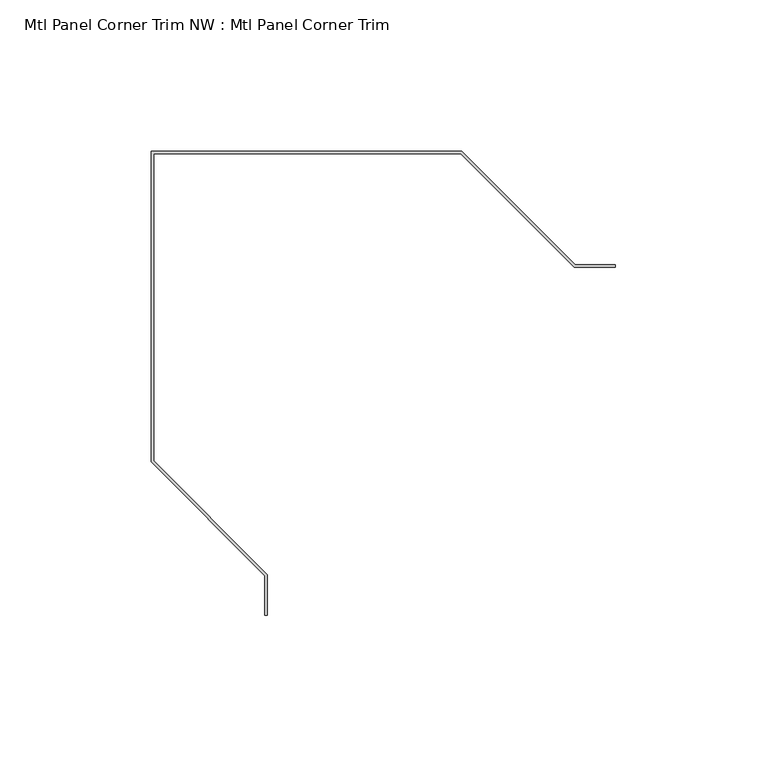
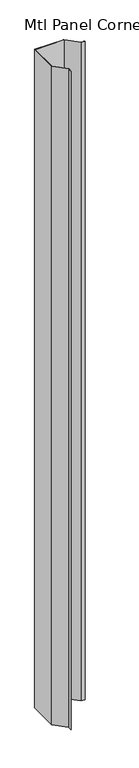
"""IFC4 building model written with IfcOpenShell, lengths in millimetres: proxy geometry, Mtl Panel Corner Trim NW : Mtl Panel Corner Trim."""

from ifc_helpers import new_model, si_unit, frame, origin, place, context, project, spatial, polyline, outline, extrude, source, transform, mapped, element, save


def mtl_panel_corner_trim_nw_mtl_panel_corner_trim_15613486(model_context):
    return source(origin(), model_context, "Body", "SweptSolid", [
        extrude(outline(polyline([(587365.3854739, -531753.7703841), (587364.5980739, -531753.7703841), (587364.5980739, -531740.6345358), (587327.0060739, -531703.0425358), (587327.0060739, -531600.3289841), (587429.7196257, -531600.3289841), (587467.2100257, -531637.8193841), (587480.4474739, -531637.8193841), (587480.4474739, -531638.6131341), (587466.8812437, -531638.6131341), (587429.3908437, -531601.1227341), (587327.7998239, -531601.1227341), (587327.7998239, -531702.7137538), (587365.3854739, -531740.2994038), (587365.3854739, -531753.7703841)])), frame((0.0, 0.0, 6.35), z_axis=(0.0, 0.0, 1.0), x_axis=(1.0, 0.0, 0.0)), (0.0, 0.0, 1.0), 2432.05),
    ])


if __name__ == "__main__":
    model = new_model("IFC4")
    model_context = context("Model", 3, world=origin())
    ifc_project = project(units=[si_unit("LENGTHUNIT", "METRE", prefix="MILLI")], contexts=[model_context])
    site = spatial("IfcSite", under=ifc_project)
    building = spatial("IfcBuilding", under=site)
    placement = place(None, origin())
    mtl_panel_corner_trim_nw_mtl_panel_corner_trim_shape = mtl_panel_corner_trim_nw_mtl_panel_corner_trim_15613486(model_context)
    element("IfcBuildingElementProxy", 1, Name="Mtl Panel Corner Trim NW : Mtl Panel Corner Trim", ObjectType="Mtl Panel Corner Trim NW : Mtl Panel Corner Trim", at=placement, inside=building, context=model_context, shape_type="MappedRepresentation", body=[
        mapped(mtl_panel_corner_trim_nw_mtl_panel_corner_trim_shape, transform((0.0, 0.0, 0.0), x_axis=(1.0, 0.0, 0.0), y_axis=(0.0, 1.0, 0.0), z_axis=(0.0, 0.0, 1.0))),
    ])
    save(model, "model.ifc")

# Revit data of these elements
# Element 1 (IfcBuildingElementProxy, "Mtl Panel Corner Trim NW : Mtl Panel Corner Trim")
#   Materials on its faces: "CORNER TRIM BY MTL PANEL MFR."
# Materials
#   "CORNER TRIM BY MTL PANEL MFR.": class "Generic", colour RGB 239 242 240, transparency 0, Cost = 0
